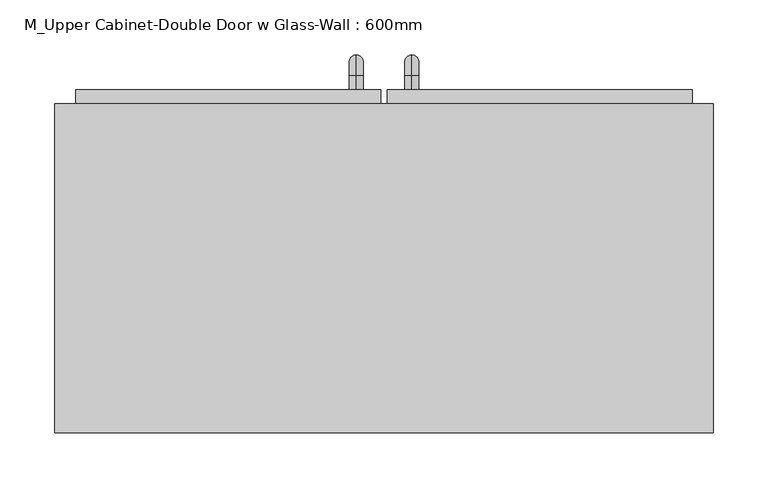
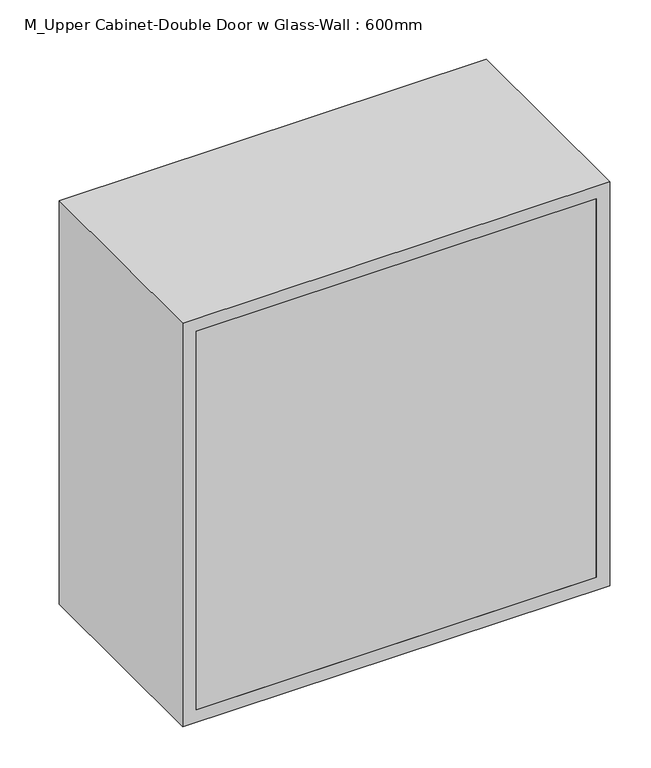
"""IFC4 building model written with IfcOpenShell, lengths in millimetres: furniture geometry, M_Upper Cabinet-Double Door w Glass-Wall : 600mm."""

from ifc_helpers import new_model, si_unit, point, frame, origin, place, context, project, spatial, polyline, circle_curve, ellipse_curve, trimmed, outline, extrude, source, transform, mapped, element, save
from ifc_brep_helpers import plane_surface, cylinder_surface, revolved_surface, advanced_brep


def m_upper_cabinet_double_door_w_glass_wall_600mm_b64e571c(model_context):
    return source(origin(), model_context, "Body", "SolidModel", [
        advanced_brep(
        [(55.1711628, 387.7, 1546.05), (55.1711628, 387.7, 1558.75), (55.1711628, 400.4, 1546.05), (55.1711628, 400.4, 1558.75), (55.1711628, 419.45, 1539.7), (55.1711628, 406.75, 1539.7), (55.1711628, 406.75, 1463.5), (55.1711628, 419.45, 1463.5), (55.1711628, 400.4, 1444.45), (55.1711628, 400.4, 1457.15), (55.1711628, 387.7, 1457.15), (55.1711628, 387.7, 1444.45)],
        [
            (0, 1, circle_curve(frame((55.1711628, 387.7, 1552.4), z_axis=(0.0, -1.0, 0.0), x_axis=(0.0, 0.0, -1.0)), 6.35)),
            (1, 0, circle_curve(frame((55.1711628, 387.7, 1552.4), z_axis=(0.0, -1.0, 0.0), x_axis=(0.0, 0.0, -1.0)), 6.35)),
            (0, 2),
            (2, 3, circle_curve(frame((55.1711628, 400.4, 1552.4), z_axis=(0.0, -1.0, 0.0), x_axis=(0.0, 0.0, -1.0)), 6.35)),
            (3, 1),
            (3, 2, circle_curve(frame((55.1711628, 400.4, 1552.4), z_axis=(0.0, -1.0, 0.0), x_axis=(0.0, 0.0, -1.0)), 6.35)),
            (4, 3, circle_curve(frame((55.1711628, 400.4, 1539.7), z_axis=(1.0, 0.0, 0.0), x_axis=(0.0, 0.0, 1.0)), 19.05)),
            (2, 5, circle_curve(frame((55.1711628, 400.4, 1539.7), z_axis=(-1.0, 0.0, 0.0), x_axis=(0.0, 0.0, 1.0)), 6.35)),
            (5, 4, circle_curve(frame((55.1711628, 413.1, 1539.7), z_axis=(0.0, 0.0, 1.0), x_axis=(0.0, -1.0, 0.0)), 6.35)),
            (4, 5, circle_curve(frame((55.1711628, 413.1, 1539.7), z_axis=(0.0, 0.0, 1.0), x_axis=(0.0, -1.0, 0.0)), 6.35)),
            (5, 6),
            (6, 7, circle_curve(frame((55.1711628, 413.1, 1463.5), z_axis=(0.0, 0.0, 1.0), x_axis=(0.0, -1.0, 0.0)), 6.35)),
            (7, 4),
            (7, 6, circle_curve(frame((55.1711628, 413.1, 1463.5), z_axis=(0.0, 0.0, 1.0), x_axis=(0.0, -1.0, 0.0)), 6.35)),
            (8, 7, circle_curve(frame((55.1711628, 400.4, 1463.5), z_axis=(1.0, 0.0, 0.0), x_axis=(0.0, 1.0, 0.0)), 19.05)),
            (6, 9, circle_curve(frame((55.1711628, 400.4, 1463.5), z_axis=(-1.0, 0.0, 0.0), x_axis=(0.0, 1.0, 0.0)), 6.35)),
            (9, 8, circle_curve(frame((55.1711628, 400.4, 1450.8), z_axis=(0.0, 1.0, 0.0), x_axis=(0.0, 0.0, 1.0)), 6.35)),
            (8, 9, circle_curve(frame((55.1711628, 400.4, 1450.8), z_axis=(0.0, 1.0, 0.0), x_axis=(0.0, 0.0, 1.0)), 6.35)),
            (10, 11, circle_curve(frame((55.1711628, 387.7, 1450.8), z_axis=(0.0, -1.0, 0.0), x_axis=(0.0, 0.0, 1.0)), 6.35)),
            (11, 10, circle_curve(frame((55.1711628, 387.7, 1450.8), z_axis=(0.0, -1.0, 0.0), x_axis=(0.0, 0.0, 1.0)), 6.35)),
            (9, 10),
            (11, 8),
        ],
        [
            plane_surface(frame((48.8211628, 387.7, 1552.4), z_axis=(0.0, -1.0, 0.0), x_axis=(0.0, 0.0, 1.0))),
            cylinder_surface(frame((55.1711628, 387.7, 1552.4), z_axis=(0.0, -1.0, 0.0), x_axis=(0.0, 0.0, -1.0)), 6.35),
            revolved_surface(trimmed(ellipse_curve(frame((55.1711628, 400.4, 1552.4), z_axis=(0.0, -1.0, 0.0), x_axis=(0.0, 0.0, -1.0)), 6.35, 6.35), [point((55.1711628, 400.4, 1546.05))], [point((55.1711628, 400.4, 1558.75))], True, "CARTESIAN"), (55.1711628, 400.4, 1539.7), (-1.0, 0.0, 0.0)),
            revolved_surface(trimmed(ellipse_curve(frame((55.1711628, 400.4, 1552.4), z_axis=(0.0, -1.0, 0.0), x_axis=(0.0, 0.0, -1.0)), 6.35, 6.35), [point((55.1711628, 400.4, 1558.75))], [point((55.1711628, 400.4, 1546.05))], True, "CARTESIAN"), (55.1711628, 400.4, 1539.7), (-1.0, 0.0, 0.0)),
            cylinder_surface(frame((55.1711628, 413.1, 1539.7), z_axis=(0.0, 0.0, 1.0), x_axis=(0.0, -1.0, 0.0)), 6.35),
            revolved_surface(trimmed(ellipse_curve(frame((55.1711628, 413.1, 1463.5), z_axis=(0.0, 0.0, 1.0), x_axis=(0.0, -1.0, 0.0)), 6.35, 6.35), [point((55.1711628, 406.75, 1463.5))], [point((55.1711628, 419.45, 1463.5))], True, "CARTESIAN"), (55.1711628, 400.4, 1463.5), (-1.0, 0.0, 0.0)),
            revolved_surface(trimmed(ellipse_curve(frame((55.1711628, 413.1, 1463.5), z_axis=(0.0, 0.0, 1.0), x_axis=(0.0, -1.0, 0.0)), 6.35, 6.35), [point((55.1711628, 419.45, 1463.5))], [point((55.1711628, 406.75, 1463.5))], True, "CARTESIAN"), (55.1711628, 400.4, 1463.5), (-1.0, 0.0, 0.0)),
            plane_surface(frame((48.8211628, 387.7, 1450.8), z_axis=(0.0, -1.0, 0.0), x_axis=(0.0, 0.0, -1.0))),
            cylinder_surface(frame((55.1711628, 400.4, 1450.8), z_axis=(0.0, 1.0, 0.0), x_axis=(0.0, 0.0, 1.0)), 6.35),
        ],
        [
            (0, [[1, 2]]),
            (1, [[-1, 3, 4, 5]]),
            (1, [[-2, -5, 6, -3]]),
            (2, [[7, -4, 8, 9]]),
            (3, [[-8, -6, -7, 10]]),
            (4, [[-9, 11, 12, 13]]),
            (4, [[-10, -13, 14, -11]]),
            (5, [[15, -12, 16, 17]]),
            (6, [[-16, -14, -15, 18]]),
            (7, [[19, 20]]),
            (8, [[-17, 21, -20, 22]]),
            (8, [[-18, -22, -19, -21]]),
        ],
    ),
        advanced_brep(
        [(4.3711628, 387.7, 1546.05), (4.3711628, 387.7, 1558.75), (4.3711628, 400.4, 1546.05), (4.3711628, 400.4, 1558.75), (4.3711628, 419.45, 1539.7), (4.3711628, 406.75, 1539.7), (4.3711628, 406.75, 1463.5), (4.3711628, 419.45, 1463.5), (4.3711628, 400.4, 1444.45), (4.3711628, 400.4, 1457.15), (4.3711628, 387.7, 1457.15), (4.3711628, 387.7, 1444.45)],
        [
            (0, 1, circle_curve(frame((4.3711628, 387.7, 1552.4), z_axis=(0.0, -1.0, 0.0), x_axis=(0.0, 0.0, 1.0)), 6.35)),
            (1, 0, circle_curve(frame((4.3711628, 387.7, 1552.4), z_axis=(0.0, -1.0, 0.0), x_axis=(0.0, 0.0, 1.0)), 6.35)),
            (0, 2),
            (2, 3, circle_curve(frame((4.3711628, 400.4, 1552.4), z_axis=(0.0, -1.0, 0.0), x_axis=(0.0, 0.0, 1.0)), 6.35)),
            (3, 1),
            (3, 2, circle_curve(frame((4.3711628, 400.4, 1552.4), z_axis=(0.0, -1.0, 0.0), x_axis=(0.0, 0.0, 1.0)), 6.35)),
            (4, 3, circle_curve(frame((4.3711628, 400.4, 1539.7), z_axis=(1.0, 0.0, 0.0), x_axis=(0.0, 0.0, 1.0)), 19.05)),
            (2, 5, circle_curve(frame((4.3711628, 400.4, 1539.7), z_axis=(-1.0, 0.0, 0.0), x_axis=(0.0, 0.0, 1.0)), 6.35)),
            (5, 4, circle_curve(frame((4.3711628, 413.1, 1539.7), z_axis=(0.0, 0.0, 1.0), x_axis=(0.0, 1.0, 0.0)), 6.35)),
            (4, 5, circle_curve(frame((4.3711628, 413.1, 1539.7), z_axis=(0.0, 0.0, 1.0), x_axis=(0.0, 1.0, 0.0)), 6.35)),
            (5, 6),
            (6, 7, circle_curve(frame((4.3711628, 413.1, 1463.5), z_axis=(0.0, 0.0, 1.0), x_axis=(0.0, 1.0, 0.0)), 6.35)),
            (7, 4),
            (7, 6, circle_curve(frame((4.3711628, 413.1, 1463.5), z_axis=(0.0, 0.0, 1.0), x_axis=(0.0, 1.0, 0.0)), 6.35)),
            (8, 7, circle_curve(frame((4.3711628, 400.4, 1463.5), z_axis=(1.0, 0.0, 0.0), x_axis=(0.0, 1.0, 0.0)), 19.05)),
            (6, 9, circle_curve(frame((4.3711628, 400.4, 1463.5), z_axis=(-1.0, 0.0, 0.0), x_axis=(0.0, 1.0, 0.0)), 6.35)),
            (9, 8, circle_curve(frame((4.3711628, 400.4, 1450.8), z_axis=(0.0, 1.0, 0.0), x_axis=(0.0, 0.0, -1.0)), 6.35)),
            (8, 9, circle_curve(frame((4.3711628, 400.4, 1450.8), z_axis=(0.0, 1.0, 0.0), x_axis=(0.0, 0.0, -1.0)), 6.35)),
            (10, 11, circle_curve(frame((4.3711628, 387.7, 1450.8), z_axis=(0.0, -1.0, 0.0), x_axis=(0.0, 0.0, -1.0)), 6.35)),
            (11, 10, circle_curve(frame((4.3711628, 387.7, 1450.8), z_axis=(0.0, -1.0, 0.0), x_axis=(0.0, 0.0, -1.0)), 6.35)),
            (9, 10),
            (11, 8),
        ],
        [
            plane_surface(frame((-1.9788372, 387.7, 1552.4), z_axis=(0.0, -1.0, 0.0), x_axis=(0.0, 0.0, 1.0))),
            cylinder_surface(frame((4.3711628, 387.7, 1552.4), z_axis=(0.0, -1.0, 0.0), x_axis=(0.0, 0.0, 1.0)), 6.35),
            revolved_surface(trimmed(ellipse_curve(frame((4.3711628, 400.4, 1552.4), z_axis=(0.0, -1.0, 0.0), x_axis=(0.0, 0.0, 1.0)), 6.35, 6.35), [point((4.3711628, 400.4, 1546.05))], [point((4.3711628, 400.4, 1558.75))], True, "CARTESIAN"), (4.3711628, 400.4, 1539.7), (-1.0, 0.0, 0.0)),
            revolved_surface(trimmed(ellipse_curve(frame((4.3711628, 400.4, 1552.4), z_axis=(0.0, -1.0, 0.0), x_axis=(0.0, 0.0, 1.0)), 6.35, 6.35), [point((4.3711628, 400.4, 1558.75))], [point((4.3711628, 400.4, 1546.05))], True, "CARTESIAN"), (4.3711628, 400.4, 1539.7), (-1.0, 0.0, 0.0)),
            cylinder_surface(frame((4.3711628, 413.1, 1539.7), z_axis=(0.0, 0.0, 1.0), x_axis=(0.0, 1.0, 0.0)), 6.35),
            revolved_surface(trimmed(ellipse_curve(frame((4.3711628, 413.1, 1463.5), z_axis=(0.0, 0.0, 1.0), x_axis=(0.0, 1.0, 0.0)), 6.35, 6.35), [point((4.3711628, 406.75, 1463.5))], [point((4.3711628, 419.45, 1463.5))], True, "CARTESIAN"), (4.3711628, 400.4, 1463.5), (-1.0, 0.0, 0.0)),
            revolved_surface(trimmed(ellipse_curve(frame((4.3711628, 413.1, 1463.5), z_axis=(0.0, 0.0, 1.0), x_axis=(0.0, 1.0, 0.0)), 6.35, 6.35), [point((4.3711628, 419.45, 1463.5))], [point((4.3711628, 406.75, 1463.5))], True, "CARTESIAN"), (4.3711628, 400.4, 1463.5), (-1.0, 0.0, 0.0)),
            plane_surface(frame((-1.9788372, 387.7, 1450.8), z_axis=(0.0, -1.0, 0.0), x_axis=(0.0, 0.0, -1.0))),
            cylinder_surface(frame((4.3711628, 400.4, 1450.8), z_axis=(0.0, 1.0, 0.0), x_axis=(0.0, 0.0, -1.0)), 6.35),
        ],
        [
            (0, [[1, 2]]),
            (1, [[-1, 3, 4, 5]]),
            (1, [[-2, -5, 6, -3]]),
            (2, [[7, -4, 8, 9]]),
            (3, [[-8, -6, -7, 10]]),
            (4, [[-9, 11, 12, 13]]),
            (4, [[-10, -13, 14, -11]]),
            (5, [[15, -12, 16, 17]]),
            (6, [[-16, -14, -15, 18]]),
            (7, [[19, 20]]),
            (8, [[-17, 21, -20, 22]]),
            (8, [[-18, -22, -19, -21]]),
        ],
    ),
        extrude(outline(polyline([(64.6961628, 368.65), (278.9711628, 368.65), (278.9711628, 362.3), (64.6961628, 362.3), (64.6961628, 368.65)])), frame((0.0, 0.0, 1450.8), z_axis=(0.0, 0.0, 1.0), x_axis=(1.0, 0.0, 0.0)), (0.0, 0.0, 1.0), 498.4),
        extrude(outline(polyline([(-219.4288372, 368.65), (-5.1538372, 368.65), (-5.1538372, 362.3), (-219.4288372, 362.3), (-219.4288372, 368.65)])), frame((0.0, 0.0, 1450.8), z_axis=(0.0, 0.0, 1.0), x_axis=(1.0, 0.0, 0.0)), (0.0, 0.0, 1.0), 498.4),
        extrude(outline(polyline([(1980.95, 32.9461628), (1419.05, 32.9461628), (1419.05, 310.7211628), (1980.95, 310.7211628), (1980.95, 32.9461628)]), holes=[polyline([(1450.8, 64.6961628), (1949.2, 64.6961628), (1949.2, 278.9711628), (1450.8, 278.9711628), (1450.8, 64.6961628)])]), frame((0.0, 355.95, 0.0), z_axis=(0.0, 1.0, 0.0), x_axis=(0.0, 0.0, 1.0)), (0.0, 0.0, 1.0), 31.75),
        extrude(outline(polyline([(1419.05, -251.1788372), (1419.05, 26.5961628), (1980.95, 26.5961628), (1980.95, -251.1788372), (1419.05, -251.1788372)]), holes=[polyline([(1949.2, -5.1538372), (1450.8, -5.1538372), (1450.8, -219.4288372), (1949.2, -219.4288372), (1949.2, -5.1538372)])]), frame((0.0, 355.95, 0.0), z_axis=(0.0, 1.0, 0.0), x_axis=(0.0, 0.0, 1.0)), (0.0, 0.0, 1.0), 31.75),
        extrude(outline(polyline([(310.7211628, 75.0), (-251.1788372, 75.0), (-251.1788372, 94.05), (310.7211628, 94.05), (310.7211628, 75.0)])), frame((0.0, 0.0, 1419.05), z_axis=(0.0, 0.0, 1.0), x_axis=(1.0, 0.0, 0.0)), (0.0, 0.0, 1.0), 561.9),
        extrude(outline(polyline([(2000.0, -270.2288372), (1400.0, -270.2288372), (1400.0, 329.7711628), (2000.0, 329.7711628), (2000.0, -270.2288372)]), holes=[polyline([(1980.95, -251.1788372), (1980.95, 310.7211628), (1419.05, 310.7211628), (1419.05, -251.1788372), (1980.95, -251.1788372)])]), frame((0.0, 75.0, 0.0), z_axis=(0.0, 1.0, 0.0), x_axis=(0.0, 0.0, 1.0)), (0.0, 0.0, 1.0), 300.0),
    ])


if __name__ == "__main__":
    model = new_model("IFC4")
    model_context = context("Model", 3, world=origin())
    ifc_project = project(units=[si_unit("LENGTHUNIT", "METRE", prefix="MILLI")], contexts=[model_context])
    site = spatial("IfcSite", under=ifc_project)
    building = spatial("IfcBuilding", under=site)
    placement = place(None, origin())
    m_upper_cabinet_double_door_w_glass_wall_600mm_shape = m_upper_cabinet_double_door_w_glass_wall_600mm_b64e571c(model_context)
    element("IfcFurniture", 1, ObjectType="M_Upper Cabinet-Double Door w Glass-Wall : 600mm", at=placement, inside=building, context=model_context, shape_type="MappedRepresentation", body=[
        mapped(m_upper_cabinet_double_door_w_glass_wall_600mm_shape, transform((0.0, 0.0, 0.0), x_axis=(1.0, 0.0, 0.0), y_axis=(0.0, 1.0, 0.0), z_axis=(0.0, 0.0, 1.0))),
    ])
    save(model, "model.ifc")

# Revit data of these elements
# Type "M_Upper Cabinet-Double Door w Glass-Wall : 600mm"
#   Depth = 0.3 m
#   Height = 0.6 m
#   Top Of Cabinet = 2 m
#   Width = 0.6 m
#   Cabinet Material = none
#   Door/Drawer Material = none
#   Handle Material = Cabinets - Handles
#   Panel Material = Cabinets - Panel/Glass
#   Default Elevation = 0
# Element 1 (IfcFurniture, "M_Upper Cabinet-Double Door w Glass-Wall : 600mm")
#   Materials on its faces: "Cabinets", "Cabinets - Handles", "Cabinets - Panel/Glass"
# Materials
#   "Cabinets - Handles": class "Metal", colour RGB 57 57 57, transparency 0
#   "Cabinets - Panel/Glass": class "Miscellaneous", colour RGB 252 255 255, transparency 0.72
#   "Cabinets": class "Miscellaneous", colour RGB 249 249 249, transparency 0
